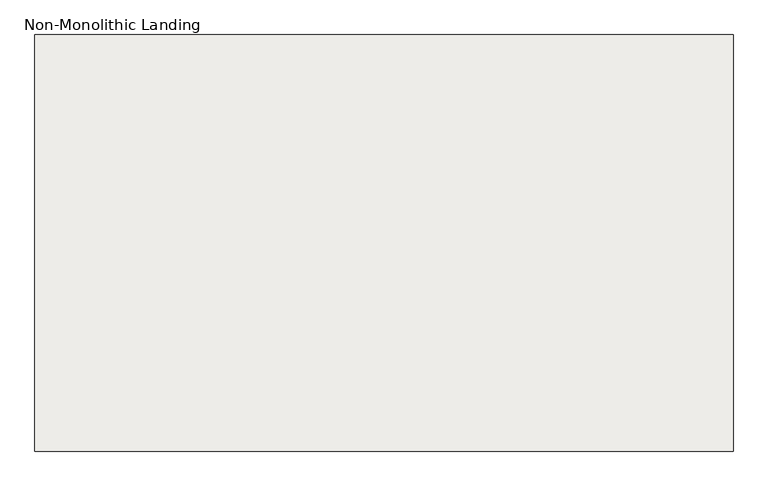
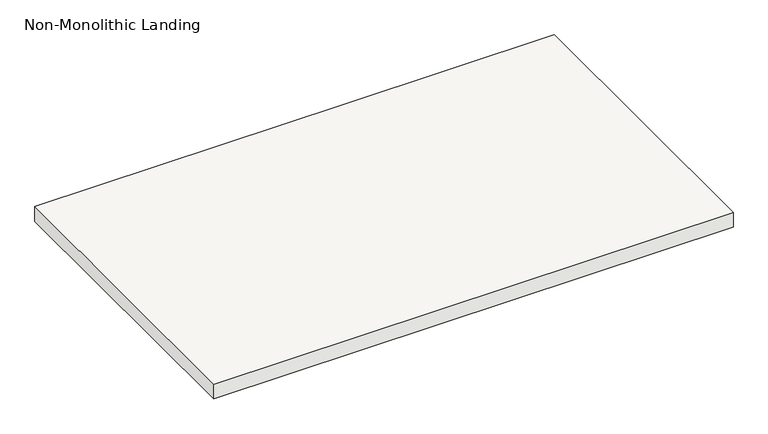
"""IFC4 building model written with IfcOpenShell, lengths in millimetres: slab geometry, Non-Monolithic Landing."""

import ifcopenshell
import ifcopenshell.guid

model = None  # the IFC model being written
_history = None  # IfcOwnerHistory: only IFC2X3 demands one
_inside = {}  # id of a spatial element -> (the spatial element, [elements in it])
_under = {}  # id of a project, library or spatial element -> (it, [spatial elements below it])
_declared = {}  # id of a project -> (the project, [libraries it declares])
_typed = {}  # id of a type object -> (the type object, [elements of that type])
_made_of = {}  # id of a material, layer set ... -> (it, [elements and type objects made of it])


def new_model(schema):
    """Start an empty IFC model of exactly this schema.

    Asked for "IFC4X3", IfcOpenShell would pick the latest addendum, in which some entities
    have other attributes; the version numbers below select the first issue.
    IFC2X3 requires an IfcOwnerHistory on every rooted entity: one is made here for all.
    """
    global model, _history
    if schema == "IFC4X3":
        model = ifcopenshell.file(schema_version=(4, 3, 0, 0))
    else:
        model = ifcopenshell.file(schema=schema)
    _inside.clear()
    _under.clear()
    _declared.clear()
    _typed.clear()
    _made_of.clear()
    _history = None
    if model.schema == "IFC2X3":
        org = make("IfcOrganization", Name="unknown")
        user = make(
            "IfcPersonAndOrganization",
            ThePerson=make("IfcPerson", FamilyName="unknown"),
            TheOrganization=org,
        )
        app = make(
            "IfcApplication",
            ApplicationDeveloper=org,
            Version="unknown",
            ApplicationFullName="unknown",
            ApplicationIdentifier="unknown",
        )
        _history = make(
            "IfcOwnerHistory",
            OwningUser=user,
            OwningApplication=app,
            ChangeAction="ADDED",
            CreationDate=0,
        )
    return model


def make(cls, **values):
    """One entity of the class cls with the attributes given. An attribute that is None is left unset."""
    return model.create_entity(
        cls, **{name: value for name, value in values.items() if value is not None}
    )


def rooted(cls, **values):
    """An entity with a GlobalId (a new one), such as an element, a storey or a relation."""
    return make(cls, GlobalId=ifcopenshell.guid.new(), OwnerHistory=_history, **values)


def si_unit(unit_type, name, prefix=None):
    """IfcSIUnit, for example si_unit("LENGTHUNIT", "METRE", prefix="MILLI")."""
    return make("IfcSIUnit", UnitType=unit_type, Prefix=prefix, Name=name)


def assignment(units):
    """IfcUnitAssignment: the units of a project."""
    return None if units is None else make("IfcUnitAssignment", Units=units)


def point(xyz):
    """IfcCartesianPoint."""
    return None if xyz is None else make("IfcCartesianPoint", Coordinates=xyz)


def direction(xyz):
    """IfcDirection."""
    return None if xyz is None else make("IfcDirection", DirectionRatios=xyz)


def frame(location, z_axis=None, x_axis=None):
    """IfcAxis2Placement3D, a coordinate frame: its origin and axes. An axis left out is left unset."""
    return make(
        "IfcAxis2Placement3D",
        Location=point(location),
        Axis=direction(z_axis),
        RefDirection=direction(x_axis),
    )


def origin():
    """The frame at (0, 0, 0) with its axes left unset."""
    return frame((0.0, 0.0, 0.0))


def place(relative_to, where):
    """IfcLocalPlacement: puts the frame where relative to a parent placement (None: the world)."""
    return make(
        "IfcLocalPlacement", PlacementRelTo=relative_to, RelativePlacement=where
    )


def context(
    kind, dimensions, precision=None, world=None, true_north=None, identifier=None
):
    """IfcGeometricRepresentationContext, for example the 3D "Model" context."""
    return make(
        "IfcGeometricRepresentationContext",
        ContextIdentifier=identifier,
        ContextType=kind,
        CoordinateSpaceDimension=dimensions,
        Precision=precision,
        WorldCoordinateSystem=world,
        TrueNorth=true_north,
    )


def project(units=None, contexts=None):
    """IfcProject with its units and contexts."""
    return rooted(
        "IfcProject",
        Name="project",
        RepresentationContexts=contexts,
        UnitsInContext=assignment(units),
    )


def spatial(cls, under=None, at=None, **own):
    """A site, building, storey or space (cls), placed at a placement, below another one or the project."""
    s = rooted(cls, ObjectPlacement=at, **own)
    if under is not None:
        _under.setdefault(under.id(), (under, []))[1].append(s)
    return s


def polyline(points):
    """IfcPolyline through the points."""
    return make("IfcPolyline", Points=[point(p) for p in points])


def outline(outer, holes=None, kind="AREA"):
    """IfcArbitraryClosedProfileDef: a profile drawn as a closed curve; with holes, ...WithVoids."""
    if holes is None:
        return make("IfcArbitraryClosedProfileDef", ProfileType=kind, OuterCurve=outer)
    return make(
        "IfcArbitraryProfileDefWithVoids",
        ProfileType=kind,
        OuterCurve=outer,
        InnerCurves=holes,
    )


def extrude(swept, where, along, depth):
    """IfcExtrudedAreaSolid: the profile swept, set in the frame where, extruded along a direction by depth."""
    return make(
        "IfcExtrudedAreaSolid",
        SweptArea=swept,
        Position=where,
        ExtrudedDirection=direction(along),
        Depth=depth,
    )


def shape(context_of_items, identifier, shape_type, items):
    """IfcShapeRepresentation: the items that make up one representation, for example the "Body"."""
    return make(
        "IfcShapeRepresentation",
        ContextOfItems=context_of_items,
        RepresentationIdentifier=identifier,
        RepresentationType=shape_type,
        Items=items,
    )


def source(mapping_origin, context_of_items, identifier, shape_type, items):
    """IfcRepresentationMap: a shape defined once, which mapped items show again and again."""
    return make(
        "IfcRepresentationMap",
        MappingOrigin=mapping_origin,
        MappedRepresentation=shape(context_of_items, identifier, shape_type, items),
    )


def transform(
    local_origin,
    x_axis=None,
    y_axis=None,
    z_axis=None,
    scale=None,
    scale2=None,
    scale3=None,
    uniform=True,
):
    """IfcCartesianTransformationOperator3D, or its non-uniform kind. x_axis, y_axis, z_axis: its Axis1, 2, 3."""
    if uniform:
        return make(
            "IfcCartesianTransformationOperator3D",
            Axis1=direction(x_axis),
            Axis2=direction(y_axis),
            LocalOrigin=point(local_origin),
            Scale=scale,
            Axis3=direction(z_axis),
        )
    return make(
        "IfcCartesianTransformationOperator3DnonUniform",
        Axis1=direction(x_axis),
        Axis2=direction(y_axis),
        LocalOrigin=point(local_origin),
        Scale=scale,
        Axis3=direction(z_axis),
        Scale2=scale2,
        Scale3=scale3,
    )


def mapped(mapping_source, mapping_target):
    """IfcMappedItem: shows the shape of a source again, moved by a transform."""
    return make(
        "IfcMappedItem", MappingSource=mapping_source, MappingTarget=mapping_target
    )


def made_of(thing, what):
    """Note that an element or type object is made of a material, layer set ...; save() writes the relation."""
    if what is not None:
        _made_of.setdefault(what.id(), (what, []))[1].append(thing)
    return thing


def element(
    cls,
    number,
    at=None,
    inside=None,
    cuts=None,
    type_object=None,
    material=None,
    context=None,
    identifier="Body",
    shape_type=None,
    held_by="IfcProductDefinitionShape",
    body=None,
    shapes=None,
    **own,
):
    """One element of the class cls, such as IfcWall. Its Tag is "e" and its number.

    at: its placement. inside: the storey or other place that contains it. cuts: it is an
    opening in that element (IfcRelVoidsElement). A single representation is given by context,
    identifier, shape_type and body (its items); several are given by shapes. held_by: the class
    of the entity that holds the representations. save() writes the other relations.
    """
    e = rooted(cls, Tag="e%d" % number, ObjectPlacement=at, **own)
    if body is not None:
        shapes = [shape(context, identifier, shape_type, body)]
    if shapes is not None:
        e.Representation = make(held_by, Representations=shapes)
    if inside is not None:
        _inside.setdefault(inside.id(), (inside, []))[1].append(e)
    if cuts is not None:
        rooted(
            "IfcRelVoidsElement", RelatingBuildingElement=cuts, RelatedOpeningElement=e
        )
    if type_object is not None:
        _typed.setdefault(type_object.id(), (type_object, []))[1].append(e)
    return made_of(e, material)


def aggregate(whole, parts):
    """IfcRelAggregates: a whole, such as a stair, and the parts it consists of."""
    return rooted("IfcRelAggregates", RelatingObject=whole, RelatedObjects=parts)


def save(model, path):
    """Write the relations noted so far, then the file.

    IfcRelAggregates (storeys below a building ...), IfcRelContainedInSpatialStructure (elements
    in a storey), IfcRelDefinesByType, IfcRelAssociatesMaterial and IfcRelDeclares: one each for
    every whole, place, type object, material and project.
    """
    for whole, parts in _under.values():
        aggregate(whole, parts)
    for where, things in _inside.values():
        rooted(
            "IfcRelContainedInSpatialStructure",
            RelatedElements=things,
            RelatingStructure=where,
        )
    for kind, things in _typed.values():
        rooted("IfcRelDefinesByType", RelatedObjects=things, RelatingType=kind)
    for what, things in _made_of.values():
        rooted("IfcRelAssociatesMaterial", RelatedObjects=things, RelatingMaterial=what)
    for by, libraries in _declared.values():
        rooted("IfcRelDeclares", RelatingContext=by, RelatedDefinitions=libraries)
    model.write(path)


def non_monolithic_landing_c5efd80b(model_context):
    return source(origin(), model_context, "Body", "SweptSolid", [
        extrude(outline(polyline([(-12626.101437, -2240.1378151), (-11950.3449834, -2240.1378151), (-11950.3449834, -3240.1378151), (-13626.101437, -3240.1378151), (-13626.101437, -2240.1378151), (-12626.101437, -2240.1378151)])), frame((0.0, 0.0, 1859.0909091), z_axis=(0.0, 0.0, 1.0), x_axis=(1.0, 0.0, 0.0)), (0.0, 0.0, 1.0), 50.0),
    ])


if __name__ == "__main__":
    model = new_model("IFC4")
    model_context = context("Model", 3, world=origin())
    ifc_project = project(units=[si_unit("LENGTHUNIT", "METRE", prefix="MILLI")], contexts=[model_context])
    site = spatial("IfcSite", under=ifc_project)
    building = spatial("IfcBuilding", under=site)
    placement = place(None, origin())
    non_monolithic_landing_shape = non_monolithic_landing_c5efd80b(model_context)
    element("IfcSlab", 1, ObjectType="Non-Monolithic Landing", at=placement, inside=building, context=model_context, shape_type="MappedRepresentation", body=[
        mapped(non_monolithic_landing_shape, transform((0.0, 0.0, 0.0), x_axis=(1.0, 0.0, 0.0), y_axis=(0.0, 1.0, 0.0), z_axis=(0.0, 0.0, 1.0))),
    ])
    save(model, "model.ifc")
